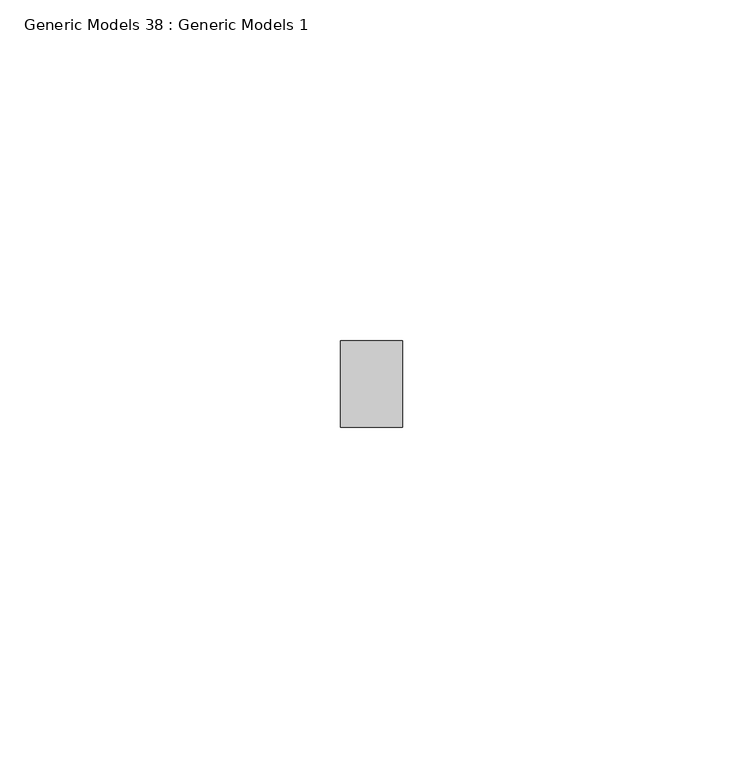
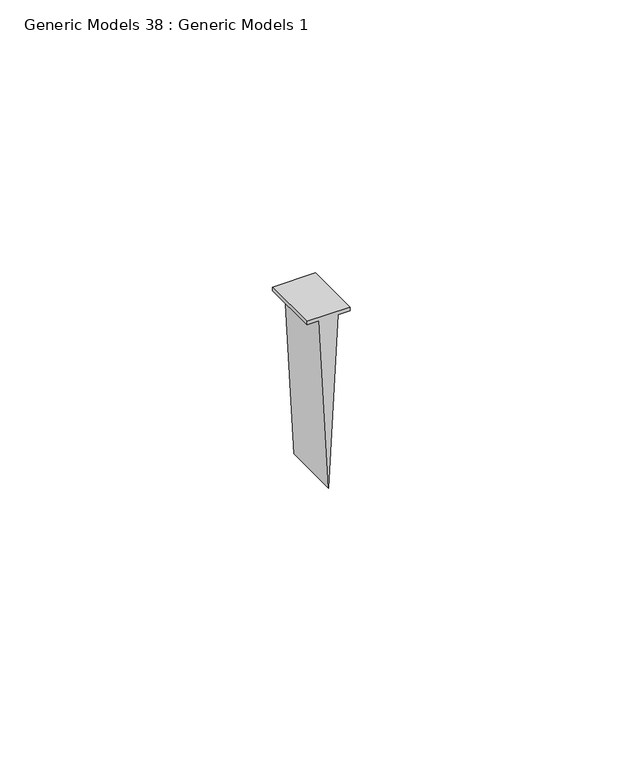
"""IFC4 building model written with IfcOpenShell, lengths in millimetres: proxy geometry, Generic Models 38 : Generic Models 1."""

import ifcopenshell
import ifcopenshell.guid

model = None  # the IFC model being written
_history = None  # IfcOwnerHistory: only IFC2X3 demands one
_inside = {}  # id of a spatial element -> (the spatial element, [elements in it])
_under = {}  # id of a project, library or spatial element -> (it, [spatial elements below it])
_declared = {}  # id of a project -> (the project, [libraries it declares])
_typed = {}  # id of a type object -> (the type object, [elements of that type])
_made_of = {}  # id of a material, layer set ... -> (it, [elements and type objects made of it])


def new_model(schema):
    """Start an empty IFC model of exactly this schema.

    Asked for "IFC4X3", IfcOpenShell would pick the latest addendum, in which some entities
    have other attributes; the version numbers below select the first issue.
    IFC2X3 requires an IfcOwnerHistory on every rooted entity: one is made here for all.
    """
    global model, _history
    if schema == "IFC4X3":
        model = ifcopenshell.file(schema_version=(4, 3, 0, 0))
    else:
        model = ifcopenshell.file(schema=schema)
    _inside.clear()
    _under.clear()
    _declared.clear()
    _typed.clear()
    _made_of.clear()
    _history = None
    if model.schema == "IFC2X3":
        org = make("IfcOrganization", Name="unknown")
        user = make(
            "IfcPersonAndOrganization",
            ThePerson=make("IfcPerson", FamilyName="unknown"),
            TheOrganization=org,
        )
        app = make(
            "IfcApplication",
            ApplicationDeveloper=org,
            Version="unknown",
            ApplicationFullName="unknown",
            ApplicationIdentifier="unknown",
        )
        _history = make(
            "IfcOwnerHistory",
            OwningUser=user,
            OwningApplication=app,
            ChangeAction="ADDED",
            CreationDate=0,
        )
    return model


def make(cls, **values):
    """One entity of the class cls with the attributes given. An attribute that is None is left unset."""
    return model.create_entity(
        cls, **{name: value for name, value in values.items() if value is not None}
    )


def rooted(cls, **values):
    """An entity with a GlobalId (a new one), such as an element, a storey or a relation."""
    return make(cls, GlobalId=ifcopenshell.guid.new(), OwnerHistory=_history, **values)


def si_unit(unit_type, name, prefix=None):
    """IfcSIUnit, for example si_unit("LENGTHUNIT", "METRE", prefix="MILLI")."""
    return make("IfcSIUnit", UnitType=unit_type, Prefix=prefix, Name=name)


def assignment(units):
    """IfcUnitAssignment: the units of a project."""
    return None if units is None else make("IfcUnitAssignment", Units=units)


def point(xyz):
    """IfcCartesianPoint."""
    return None if xyz is None else make("IfcCartesianPoint", Coordinates=xyz)


def direction(xyz):
    """IfcDirection."""
    return None if xyz is None else make("IfcDirection", DirectionRatios=xyz)


def frame(location, z_axis=None, x_axis=None):
    """IfcAxis2Placement3D, a coordinate frame: its origin and axes. An axis left out is left unset."""
    return make(
        "IfcAxis2Placement3D",
        Location=point(location),
        Axis=direction(z_axis),
        RefDirection=direction(x_axis),
    )


def origin():
    """The frame at (0, 0, 0) with its axes left unset."""
    return frame((0.0, 0.0, 0.0))


def place(relative_to, where):
    """IfcLocalPlacement: puts the frame where relative to a parent placement (None: the world)."""
    return make(
        "IfcLocalPlacement", PlacementRelTo=relative_to, RelativePlacement=where
    )


def context(
    kind, dimensions, precision=None, world=None, true_north=None, identifier=None
):
    """IfcGeometricRepresentationContext, for example the 3D "Model" context."""
    return make(
        "IfcGeometricRepresentationContext",
        ContextIdentifier=identifier,
        ContextType=kind,
        CoordinateSpaceDimension=dimensions,
        Precision=precision,
        WorldCoordinateSystem=world,
        TrueNorth=true_north,
    )


def project(units=None, contexts=None):
    """IfcProject with its units and contexts."""
    return rooted(
        "IfcProject",
        Name="project",
        RepresentationContexts=contexts,
        UnitsInContext=assignment(units),
    )


def spatial(cls, under=None, at=None, **own):
    """A site, building, storey or space (cls), placed at a placement, below another one or the project."""
    s = rooted(cls, ObjectPlacement=at, **own)
    if under is not None:
        _under.setdefault(under.id(), (under, []))[1].append(s)
    return s


def polyline(points):
    """IfcPolyline through the points."""
    return make("IfcPolyline", Points=[point(p) for p in points])


def outline(outer, holes=None, kind="AREA"):
    """IfcArbitraryClosedProfileDef: a profile drawn as a closed curve; with holes, ...WithVoids."""
    if holes is None:
        return make("IfcArbitraryClosedProfileDef", ProfileType=kind, OuterCurve=outer)
    return make(
        "IfcArbitraryProfileDefWithVoids",
        ProfileType=kind,
        OuterCurve=outer,
        InnerCurves=holes,
    )


def extrude(swept, where, along, depth):
    """IfcExtrudedAreaSolid: the profile swept, set in the frame where, extruded along a direction by depth."""
    return make(
        "IfcExtrudedAreaSolid",
        SweptArea=swept,
        Position=where,
        ExtrudedDirection=direction(along),
        Depth=depth,
    )


def shape(context_of_items, identifier, shape_type, items):
    """IfcShapeRepresentation: the items that make up one representation, for example the "Body"."""
    return make(
        "IfcShapeRepresentation",
        ContextOfItems=context_of_items,
        RepresentationIdentifier=identifier,
        RepresentationType=shape_type,
        Items=items,
    )


def source(mapping_origin, context_of_items, identifier, shape_type, items):
    """IfcRepresentationMap: a shape defined once, which mapped items show again and again."""
    return make(
        "IfcRepresentationMap",
        MappingOrigin=mapping_origin,
        MappedRepresentation=shape(context_of_items, identifier, shape_type, items),
    )


def transform(
    local_origin,
    x_axis=None,
    y_axis=None,
    z_axis=None,
    scale=None,
    scale2=None,
    scale3=None,
    uniform=True,
):
    """IfcCartesianTransformationOperator3D, or its non-uniform kind. x_axis, y_axis, z_axis: its Axis1, 2, 3."""
    if uniform:
        return make(
            "IfcCartesianTransformationOperator3D",
            Axis1=direction(x_axis),
            Axis2=direction(y_axis),
            LocalOrigin=point(local_origin),
            Scale=scale,
            Axis3=direction(z_axis),
        )
    return make(
        "IfcCartesianTransformationOperator3DnonUniform",
        Axis1=direction(x_axis),
        Axis2=direction(y_axis),
        LocalOrigin=point(local_origin),
        Scale=scale,
        Axis3=direction(z_axis),
        Scale2=scale2,
        Scale3=scale3,
    )


def mapped(mapping_source, mapping_target):
    """IfcMappedItem: shows the shape of a source again, moved by a transform."""
    return make(
        "IfcMappedItem", MappingSource=mapping_source, MappingTarget=mapping_target
    )


def made_of(thing, what):
    """Note that an element or type object is made of a material, layer set ...; save() writes the relation."""
    if what is not None:
        _made_of.setdefault(what.id(), (what, []))[1].append(thing)
    return thing


def element(
    cls,
    number,
    at=None,
    inside=None,
    cuts=None,
    type_object=None,
    material=None,
    context=None,
    identifier="Body",
    shape_type=None,
    held_by="IfcProductDefinitionShape",
    body=None,
    shapes=None,
    **own,
):
    """One element of the class cls, such as IfcWall. Its Tag is "e" and its number.

    at: its placement. inside: the storey or other place that contains it. cuts: it is an
    opening in that element (IfcRelVoidsElement). A single representation is given by context,
    identifier, shape_type and body (its items); several are given by shapes. held_by: the class
    of the entity that holds the representations. save() writes the other relations.
    """
    e = rooted(cls, Tag="e%d" % number, ObjectPlacement=at, **own)
    if body is not None:
        shapes = [shape(context, identifier, shape_type, body)]
    if shapes is not None:
        e.Representation = make(held_by, Representations=shapes)
    if inside is not None:
        _inside.setdefault(inside.id(), (inside, []))[1].append(e)
    if cuts is not None:
        rooted(
            "IfcRelVoidsElement", RelatingBuildingElement=cuts, RelatedOpeningElement=e
        )
    if type_object is not None:
        _typed.setdefault(type_object.id(), (type_object, []))[1].append(e)
    return made_of(e, material)


def aggregate(whole, parts):
    """IfcRelAggregates: a whole, such as a stair, and the parts it consists of."""
    return rooted("IfcRelAggregates", RelatingObject=whole, RelatedObjects=parts)


def save(model, path):
    """Write the relations noted so far, then the file.

    IfcRelAggregates (storeys below a building ...), IfcRelContainedInSpatialStructure (elements
    in a storey), IfcRelDefinesByType, IfcRelAssociatesMaterial and IfcRelDeclares: one each for
    every whole, place, type object, material and project.
    """
    for whole, parts in _under.values():
        aggregate(whole, parts)
    for where, things in _inside.values():
        rooted(
            "IfcRelContainedInSpatialStructure",
            RelatedElements=things,
            RelatingStructure=where,
        )
    for kind, things in _typed.values():
        rooted("IfcRelDefinesByType", RelatedObjects=things, RelatingType=kind)
    for what, things in _made_of.values():
        rooted("IfcRelAssociatesMaterial", RelatedObjects=things, RelatingMaterial=what)
    for by, libraries in _declared.values():
        rooted("IfcRelDeclares", RelatingContext=by, RelatedDefinitions=libraries)
    model.write(path)


def generic_models_38_generic_models_1_054f0e14(model_context):
    return source(origin(), model_context, "Body", "SweptSolid", [
        extrude(outline(polyline([(2443.027413, 49845.474547), (2442.233663, 49845.474547), (2442.233663, 49848.0244106), (2404.133663, 49850.021147), (2442.233663, 49852.0178834), (2442.233663, 49854.567747), (2443.027413, 49854.567747), (2443.027413, 49845.474547)])), frame((0.0, 565.15, 0.0), z_axis=(0.0, 1.0, 0.0), x_axis=(0.0, 0.0, 1.0)), (0.0, 0.0, 1.0), 12.7),
    ])


if __name__ == "__main__":
    model = new_model("IFC4")
    model_context = context("Model", 3, world=origin())
    ifc_project = project(units=[si_unit("LENGTHUNIT", "METRE", prefix="MILLI")], contexts=[model_context])
    site = spatial("IfcSite", under=ifc_project)
    building = spatial("IfcBuilding", under=site)
    placement = place(None, origin())
    generic_models_38_generic_models_1_shape = generic_models_38_generic_models_1_054f0e14(model_context)
    element("IfcBuildingElementProxy", 1, Name="Generic Models 38 : Generic Models 1", ObjectType="Generic Models 38 : Generic Models 1", at=placement, inside=building, context=model_context, shape_type="MappedRepresentation", body=[
        mapped(generic_models_38_generic_models_1_shape, transform((0.0, 0.0, 0.0), x_axis=(1.0, 0.0, 0.0), y_axis=(0.0, 1.0, 0.0), z_axis=(0.0, 0.0, 1.0))),
    ])
    save(model, "model.ifc")

# Revit data of these elements
# Element 1 (IfcBuildingElementProxy, "Generic Models 38 : Generic Models 1")
#   Materials on its faces: "ATTACH GYPSUM BOARD TO STUDS AND NOT TO TOP TRACK"
# Materials
#   "ATTACH GYPSUM BOARD TO STUDS AND NOT TO TOP TRACK": class "Generic", colour RGB 48 48 48, transparency 0, Cost = 0
